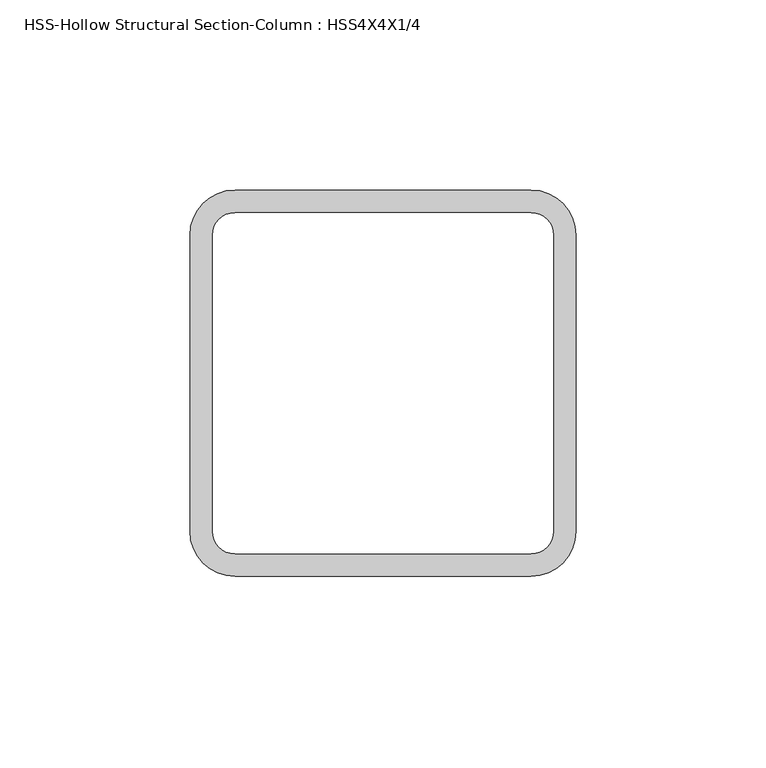
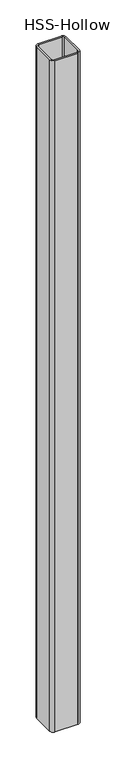
"""IFC4 building model written with IfcOpenShell, lengths in millimetres: column geometry, HSS-Hollow Structural Section-Column : HSS4X4X1/4."""

from ifc_helpers import new_model, si_unit, point, frame_2d, origin, origin_with_axes, place, context, project, spatial, polyline, circle_curve, trimmed, segment, composite_curve, outline, extrude, source, transform, mapped, element, save


def hss_hollow_structural_section_column_hss4x4x1_4_8f88891c(model_context):
    return source(origin(), model_context, "Body", "SweptSolid", [
        extrude(outline(composite_curve([segment(trimmed(circle_curve(frame_2d((38.9636, 38.9636)), 11.8364), [point((38.9636, 50.8))], [point((50.8, 38.9636))], False, "CARTESIAN"), True, "CONTINUOUS"), segment(polyline([(50.8, 38.9636), (50.8, -38.9636)]), True, "CONTINUOUS"), segment(trimmed(circle_curve(frame_2d((38.9636, -38.9636)), 11.8364), [point((50.8, -38.9636))], [point((38.9636, -50.8))], False, "CARTESIAN"), True, "CONTINUOUS"), segment(polyline([(38.9636, -50.8), (-38.9636, -50.8)]), True, "CONTINUOUS"), segment(trimmed(circle_curve(frame_2d((-38.9636, -38.9636)), 11.8364), [point((-38.9636, -50.8))], [point((-50.8, -38.9636))], False, "CARTESIAN"), True, "CONTINUOUS"), segment(polyline([(-50.8, -38.9636), (-50.8, 38.9636)]), True, "CONTINUOUS"), segment(trimmed(circle_curve(frame_2d((-38.9636, 38.9636)), 11.8364), [point((-50.8, 38.9636))], [point((-38.9636, 50.8))], False, "CARTESIAN"), True, "CONTINUOUS"), segment(polyline([(-38.9636, 50.8), (38.9636, 50.8)]), True, "CONTINUOUS")], self_intersect=False), holes=[composite_curve([segment(polyline([(38.9636, 44.8818), (-38.9636, 44.8818)]), True, "CONTINUOUS"), segment(trimmed(circle_curve(frame_2d((-38.9636, 38.9636)), 5.9182), [point((-38.9636, 44.8818))], [point((-44.8818, 38.9636))], True, "CARTESIAN"), True, "CONTINUOUS"), segment(polyline([(-44.8818, 38.9636), (-44.8818, -38.9636)]), True, "CONTINUOUS"), segment(trimmed(circle_curve(frame_2d((-38.9636, -38.9636)), 5.9182), [point((-44.8818, -38.9636))], [point((-38.9636, -44.8818))], True, "CARTESIAN"), True, "CONTINUOUS"), segment(polyline([(-38.9636, -44.8818), (38.9636, -44.8818)]), True, "CONTINUOUS"), segment(trimmed(circle_curve(frame_2d((38.9636, -38.9636)), 5.9182), [point((38.9636, -44.8818))], [point((44.8818, -38.9636))], True, "CARTESIAN"), True, "CONTINUOUS"), segment(polyline([(44.8818, -38.9636), (44.8818, 38.9636)]), True, "CONTINUOUS"), segment(trimmed(circle_curve(frame_2d((38.9636, 38.9636)), 5.9182), [point((44.8818, 38.9636))], [point((38.9636, 44.8818))], True, "CARTESIAN"), True, "CONTINUOUS")], self_intersect=False)]), origin_with_axes(), (0.0, 0.0, 1.0), 2438.4),
    ])


if __name__ == "__main__":
    model = new_model("IFC4")
    model_context = context("Model", 3, world=origin())
    ifc_project = project(units=[si_unit("LENGTHUNIT", "METRE", prefix="MILLI")], contexts=[model_context])
    site = spatial("IfcSite", under=ifc_project)
    building = spatial("IfcBuilding", under=site)
    placement = place(None, origin())
    hss_hollow_structural_section_column_hss4x4x1_4_shape = hss_hollow_structural_section_column_hss4x4x1_4_8f88891c(model_context)
    element("IfcColumn", 1, ObjectType="HSS-Hollow Structural Section-Column : HSS4X4X1/4", at=placement, inside=building, context=model_context, shape_type="MappedRepresentation", body=[
        mapped(hss_hollow_structural_section_column_hss4x4x1_4_shape, transform((0.0, 0.0, 0.0), x_axis=(1.0, 0.0, 0.0), y_axis=(0.0, 1.0, 0.0), z_axis=(0.0, 0.0, 1.0))),
    ])
    save(model, "model.ifc")

# Revit data of these elements
# Type "HSS-Hollow Structural Section-Column : HSS4X4X1/4"
#   Assembly Code = "B10"
#   Shape = "Square"
#   W = 12.2
#   Ht = 0' - 4"
#   b = 0' - 4"
#   kr = 0' - 0.466"
#   t = 0' - 0.233"
#   A = 0.0234028 SF
#   Structural Material [instance default] = 1 1/2" X 1 1/2" SPLIT-SEAM SQUARE TUBING (~24" CANTILEVER FROM C.L. OF GLULAM)
# Element 1 (IfcColumn, "HSS-Hollow Structural Section-Column : HSS4X4X1/4")
#   Structural Material = STRUCTURAL STEEL - SEE STRUCT. DWGS
#   Materials on its faces: "STRUCTURAL STEEL - SEE STRUCT. DWGS"
# Materials
#   "1 1/2\" X 1 1/2\" SPLIT-SEAM SQUARE TUBING (~24\" CANTILEVER FROM C.L. OF GLULAM)": class "Metal", colour RGB 199 199 199, transparency 0, Description = "Carbon steel", Cost = 0
#   "STRUCTURAL STEEL - SEE STRUCT. DWGS": class "Metal", colour RGB 137 146 153, transparency 0, Description = "Steel, mill finish", Cost = 0
